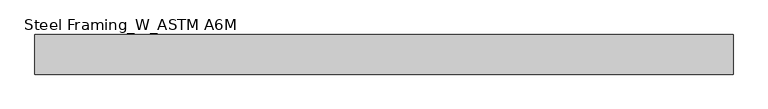
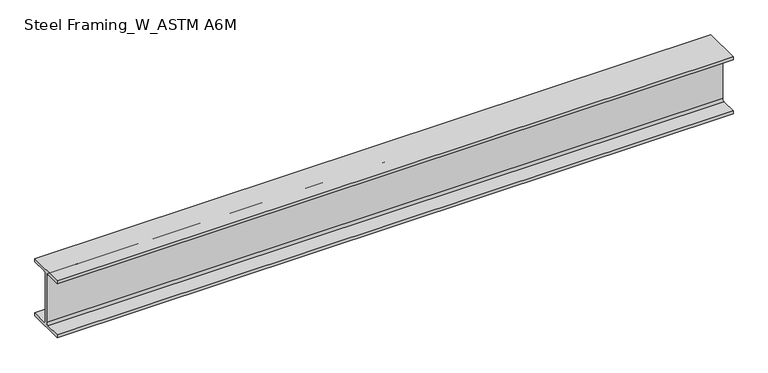
"""IFC4 building model written with IfcOpenShell, lengths in millimetres: beam geometry, Steel Framing_W_ASTM A6M : H_SB_AR_S02_W200x31.3_B6."""

from ifc_helpers import new_model, si_unit, point, frame, frame_2d, origin, place, context, project, spatial, polyline, circle_curve, trimmed, segment, composite_curve, outline, extrude, source, transform, mapped, element, save


def steel_framing_w_astm_a6m_0c2b25f3(model_context):
    return source(origin(), model_context, "Body", "SweptSolid", [
        extrude(outline(composite_curve([segment(polyline([(67.0, -94.8), (67.0, -105.0), (-67.0, -105.0), (-67.0, -94.8), (-10.775, -94.8)]), True, "CONTINUOUS"), segment(trimmed(circle_curve(frame_2d((-10.775, -87.2)), 7.6), [point((-10.775, -94.8))], [point((-3.175, -87.2))], True, "CARTESIAN"), True, "CONTINUOUS"), segment(polyline([(-3.175, -87.2), (-3.175, 87.2)]), True, "CONTINUOUS"), segment(trimmed(circle_curve(frame_2d((-10.775, 87.2)), 7.6), [point((-3.175, 87.2))], [point((-10.775, 94.8))], True, "CARTESIAN"), True, "CONTINUOUS"), segment(polyline([(-10.775, 94.8), (-67.0, 94.8), (-67.0, 105.0), (67.0, 105.0), (67.0, 94.8), (10.775, 94.8)]), True, "CONTINUOUS"), segment(trimmed(circle_curve(frame_2d((10.775, 87.2)), 7.6), [point((10.775, 94.8))], [point((3.175, 87.2))], True, "CARTESIAN"), True, "CONTINUOUS"), segment(polyline([(3.175, 87.2), (3.175, -87.2)]), True, "CONTINUOUS"), segment(trimmed(circle_curve(frame_2d((10.775, -87.2)), 7.6), [point((3.175, -87.2))], [point((10.775, -94.8))], True, "CARTESIAN"), True, "CONTINUOUS"), segment(polyline([(10.775, -94.8), (67.0, -94.8)]), True, "CONTINUOUS")], self_intersect=False)), frame((-1181.3, 0.0, 0.0), z_axis=(1.0, 0.0, 0.0), x_axis=(0.0, 1.0, 0.0)), (0.0, 0.0, 1.0), 2362.6),
    ])


if __name__ == "__main__":
    model = new_model("IFC4")
    model_context = context("Model", 3, world=origin())
    ifc_project = project(units=[si_unit("LENGTHUNIT", "METRE", prefix="MILLI")], contexts=[model_context])
    site = spatial("IfcSite", under=ifc_project)
    building = spatial("IfcBuilding", under=site)
    placement = place(None, origin())
    steel_framing_w_astm_a6m_shape = steel_framing_w_astm_a6m_0c2b25f3(model_context)
    element("IfcBeam", 1, ObjectType="Steel Framing_W_ASTM A6M : H_SB_AR_S02_W200x31.3_B6", at=placement, inside=building, context=model_context, shape_type="MappedRepresentation", body=[
        mapped(steel_framing_w_astm_a6m_shape, transform((0.0, 0.0, 0.0), x_axis=(1.0, 0.0, 0.0), y_axis=(0.0, 1.0, 0.0), z_axis=(0.0, 0.0, 1.0))),
    ])
    save(model, "model.ifc")

# Revit data of these elements
# Type "Steel Framing_W_ASTM A6M : H_SB_AR_S02_W200x31.3_B6"
#   Type Mark = "B6"
#   Section Name Key = "W8x21"
#   Width = 13.4 cm
#   Web Thickness = 0.635 cm
#   Web Fillet = 0.76 cm
#   Warping Constant = 40800.0 cm⁶
#   Torsional Moment of Inertia = 11.70 cm⁴
#   Section Area = 39.7 cm²
#   Plastic Modulus weak axis = 93.2 cm³
#   Plastic Modulus strong axis = 334.0 cm³
#   Perimeter = 0.93 m²/m
#   Nominal Weight = 31.30 kgf/m
#   Moment of Inertia weak axis = 407.00 cm⁴
#   Moment of Inertia strong axis = 3130.00 cm⁴
#   Height = 21.0 cm
#   Flange Thickness = 1.02 cm
#   Elastic Modulus weak axis = 60.8 cm³
#   Elastic Modulus strong axis = 298.0 cm³
#   Centroid Vertical = 10.5 cm
#   Centroid Horizontal = 6.7 cm
#   Length [instance default] = 1500 mm
#   Structural Material [instance default] = Steel, 45-345
#   Bolt Spacing = 0
#   Assembly Code = ""
# Element 1 (IfcBeam, "Steel Framing_W_ASTM A6M : H_SB_AR_S02_W200x31.3_B6")
#   Materials on its faces: "Steel, 45-345"
# Materials
#   "Steel, 45-345": class "Metal", colour RGB 189 187 185, transparency 0, Description = "Steel 345 MPa", Cost = 0
